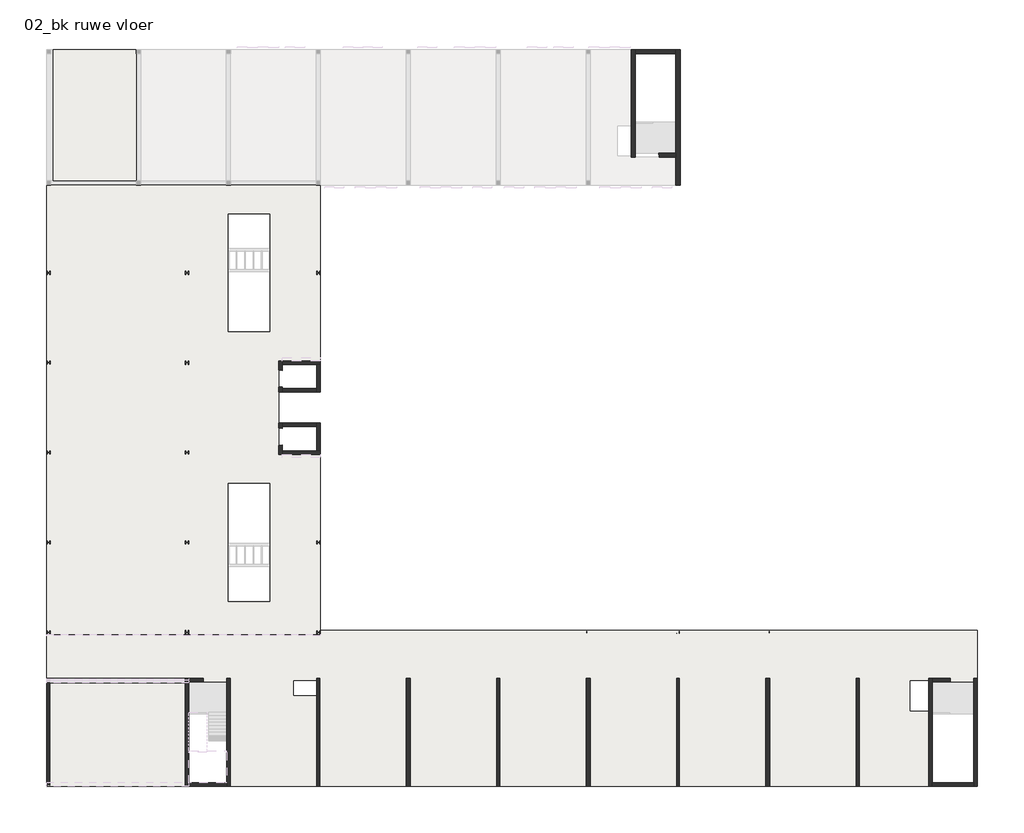
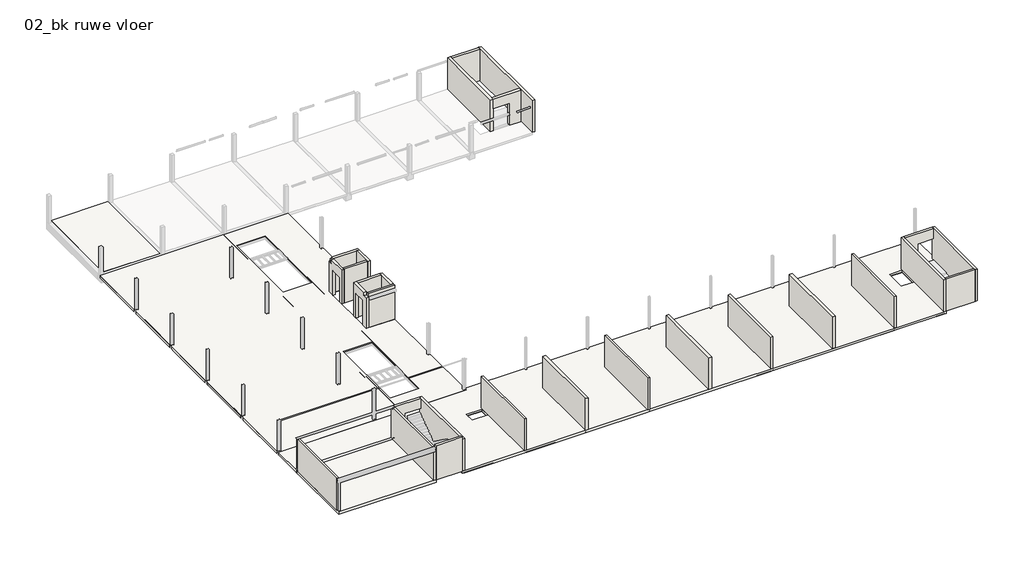
# One storey, part 1 of 3: 28 walls, 20 slabs.
"""IFC4 building model written with IfcOpenShell, lengths in millimetres."""

from ifc_helpers import new_model, si_unit, frame, origin, place, context, project, spatial, polyline, outline, extrude, faceted_brep, element, save

model = new_model("IFC4")

# Units and contexts
model_context = context("Model", 3, world=origin())
ifc_project = project(units=[si_unit("LENGTHUNIT", "METRE", prefix="MILLI")], contexts=[model_context])

# Site, building, storey
site = spatial("IfcSite", under=ifc_project)
building = spatial("IfcBuilding", under=site)
storey = spatial("IfcBuildingStorey", under=building, Name="02_bk ruwe vloer", Elevation=7530.0)

# Slabs
placement = place(None, origin())
element("IfcSlab", 1, ObjectType="NLRS_23_FL_breedplaat 260_gen_rsf", at=placement, inside=storey, context=model_context, shape_type="Brep", body=[
    faceted_brep([(70375.0, -150.0, 7270.0), (70125.0, -150.0, 7270.0), (65150.0, -150.0, 7270.0), (64850.0, -150.0, 7270.0), (58650.0, -150.0, 7270.0), (58350.0, -150.0, 7270.0), (52150.0, -150.0, 7270.0), (51850.0, -150.0, 7270.0), (45650.0, -150.0, 7270.0), (45350.0, -150.0, 7270.0), (39150.0, -150.0, 7270.0), (38850.0, -150.0, 7270.0), (32650.0, -150.0, 7270.0), (32350.0, -150.0, 7270.0), (19625.0, -150.0, 7270.0), (19375.0, -150.0, 7270.0), (19375.0, 7400.0, 7270.0), (16625.0, 7400.0, 7270.0), (16625.0, 7493.0, 7270.0), (16625.0, 7507.0, 7270.0), (6350.0, 7507.0, 7270.0), (6350.0, 10845.0, 7270.0), (26125.0, 10845.0, 7270.0), (26125.0, 11125.0, 7270.0), (73650.0, 11125.0, 7270.0), (73650.0, 7400.0, 7270.0), (73400.0, 7400.0, 7270.0), (70375.0, 7400.0, 7270.0), (6370.0, 7622.0, 7270.0), (19600.0, 7622.0, 7270.0), (19600.0, -130.0, 7270.0), (25875.0, -130.0, 7270.0), (25875.0, 7625.0, 7270.0), (26125.0, 7625.0, 7270.0), (26125.0, -130.0, 7270.0), (32375.0, -130.0, 7270.0), (32375.0, 125.0, 7270.0), (32625.0, 125.0, 7270.0), (32625.0, -130.0, 7270.0), (38875.0, -130.0, 7270.0), (38875.0, 7625.0, 7270.0), (39125.0, 7625.0, 7270.0), (39125.0, -130.0, 7270.0), (45375.0, -130.0, 7270.0), (45375.0, 125.0, 7270.0), (45625.0, 125.0, 7270.0), (45625.0, -130.0, 7270.0), (51875.0, -130.0, 7270.0), (51875.0, 7625.0, 7270.0), (52125.0, 7625.0, 7270.0), (52125.0, -130.0, 7270.0), (58375.0, -130.0, 7270.0), (58375.0, 125.0, 7270.0), (58625.0, 125.0, 7270.0), (58625.0, -130.0, 7270.0), (64875.0, -130.0, 7270.0), (64875.0, 7625.0, 7270.0), (65125.0, 7625.0, 7270.0), (65125.0, -130.0, 7270.0), (70150.0, -130.0, 7270.0), (70150.0, 7625.0, 7270.0), (73630.0, 7625.0, 7270.0), (73630.0, 11105.0, 7270.0), (26145.0, 11105.0, 7270.0), (26145.0, 10761.5, 7270.0), (6370.0, 10761.5, 7270.0), (32375.0, 7625.0, 7270.0), (32625.0, 7625.0, 7270.0), (32625.0, 7375.0, 7270.0), (32375.0, 7375.0, 7270.0), (45375.0, 7625.0, 7270.0), (45625.0, 7625.0, 7270.0), (45625.0, 7375.0, 7270.0), (45375.0, 7375.0, 7270.0), (58375.0, 7625.0, 7270.0), (58625.0, 7625.0, 7270.0), (58625.0, 7375.0, 7270.0), (58375.0, 7375.0, 7270.0), (19375.0, -150.0, 7530.0), (19625.0, -150.0, 7530.0), (32350.0, -150.0, 7530.0), (32650.0, -150.0, 7530.0), (45350.0, -150.0, 7530.0), (45650.0, -150.0, 7530.0), (58350.0, -150.0, 7530.0), (58650.0, -150.0, 7530.0), (70125.0, -150.0, 7530.0), (70375.0, -150.0, 7530.0), (70375.0, 7400.0, 7530.0), (71700.0, 7400.0, 7530.0), (73650.0, 7400.0, 7530.0), (73650.0, 11125.0, 7530.0), (26125.0, 11125.0, 7530.0), (26125.0, 10845.0, 7530.0), (6350.0, 10845.0, 7530.0), (6350.0, 7507.0, 7530.0), (16625.0, 7507.0, 7530.0), (16625.0, 7493.0, 7530.0), (16625.0, 7400.0, 7530.0), (19375.0, 7400.0, 7530.0), (19375.0, 100.0, 7530.0), (24227.5, 6452.0, 7530.0), (24227.5, 7500.0, 7530.0), (25850.0, 7500.0, 7530.0), (25850.0, 6452.0, 7530.0), (68805.0, 5320.0, 7530.0), (68805.0, 7500.0, 7530.0), (70125.0, 7500.0, 7530.0), (70125.0, 5320.0, 7530.0), (6350.0, 10845.0, 7480.0), (26125.0, 10845.0, 7480.0), (19600.0, 7622.0, 7330.0), (6370.0, 7622.0, 7330.0), (6370.0, 10761.5, 7330.0), (26145.0, 10761.5, 7330.0), (26145.0, 11105.0, 7330.0), (73630.0, 11105.0, 7330.0), (73630.0, 7625.0, 7330.0), (70150.0, 7625.0, 7330.0), (70150.0, -130.0, 7330.0), (65125.0, -130.0, 7330.0), (65125.0, 7625.0, 7330.0), (64875.0, 7625.0, 7330.0), (64875.0, -130.0, 7330.0), (58625.0, -130.0, 7330.0), (58625.0, 125.0, 7330.0), (58375.0, 125.0, 7330.0), (58375.0, -130.0, 7330.0), (52125.0, -130.0, 7330.0), (52125.0, 7625.0, 7330.0), (51875.0, 7625.0, 7330.0), (51875.0, -130.0, 7330.0), (45625.0, -130.0, 7330.0), (45625.0, 125.0, 7330.0), (45375.0, 125.0, 7330.0), (45375.0, -130.0, 7330.0), (39125.0, -130.0, 7330.0), (39125.0, 7625.0, 7330.0), (38875.0, 7625.0, 7330.0), (38875.0, -130.0, 7330.0), (32625.0, -130.0, 7330.0), (32625.0, 125.0, 7330.0), (32375.0, 125.0, 7330.0), (32375.0, -130.0, 7330.0), (26125.0, -130.0, 7330.0), (26125.0, 7625.0, 7330.0), (25875.0, 7625.0, 7330.0), (25875.0, -130.0, 7330.0), (19600.0, -130.0, 7330.0), (32625.0, 7625.0, 7330.0), (32375.0, 7625.0, 7330.0), (32375.0, 7375.0, 7330.0), (32625.0, 7375.0, 7330.0), (45625.0, 7625.0, 7330.0), (45375.0, 7625.0, 7330.0), (45375.0, 7375.0, 7330.0), (45625.0, 7375.0, 7330.0), (58625.0, 7625.0, 7330.0), (58375.0, 7625.0, 7330.0), (58375.0, 7375.0, 7330.0), (58625.0, 7375.0, 7330.0), (24227.5, 7500.0, 7330.0), (24227.5, 6452.0, 7330.0), (25850.0, 6452.0, 7330.0), (25850.0, 7500.0, 7330.0), (68805.0, 7500.0, 7330.0), (68805.0, 5320.0, 7330.0), (70125.0, 5320.0, 7330.0), (70125.0, 7500.0, 7330.0)], [[[0, 1, 2, 3, 4, 5, 6, 7, 8, 9, 10, 11, 12, 13, 14, 15, 16, 17, 18, 19, 20, 21, 22, 23, 24, 25, 26, 27], [28, 29, 30, 31, 32, 33, 34, 35, 36, 37, 38, 39, 40, 41, 42, 43, 44, 45, 46, 47, 48, 49, 50, 51, 52, 53, 54, 55, 56, 57, 58, 59, 60, 61, 62, 63, 64, 65]], [[66, 67, 68, 69]], [[70, 71, 72, 73]], [[74, 75, 76, 77]], [[78, 79, 80, 81, 82, 83, 84, 85, 86, 87, 88, 89, 90, 91, 92, 93, 94, 95, 96, 97, 98, 99, 100], [101, 102, 103, 104], [105, 106, 107, 108]], [[15, 14, 13, 12, 11, 10, 9, 8, 7, 6, 5, 4, 3, 2, 1, 0, 87, 86, 85, 84, 83, 82, 81, 80, 79, 78]], [[16, 15, 78, 100, 99]], [[17, 16, 99, 98]], [[17, 98, 97, 96, 19, 18]], [[21, 20, 95, 94, 109]], [[22, 21, 109, 94, 93, 110]], [[23, 22, 110, 93, 92]], [[24, 23, 92, 91]], [[25, 24, 91, 90]], [[27, 26, 25, 90, 89, 88]], [[0, 27, 88, 87]], [[20, 19, 96, 95]], [[111, 112, 113, 114, 115, 116, 117, 118, 119, 120, 121, 122, 123, 124, 125, 126, 127, 128, 129, 130, 131, 132, 133, 134, 135, 136, 137, 138, 139, 140, 141, 142, 143, 144, 145, 146, 147, 148], [149, 150, 151, 152], [153, 154, 155, 156], [157, 158, 159, 160], [161, 162, 163, 164], [165, 166, 167, 168]], [[112, 111, 29, 28]], [[113, 112, 28, 65]], [[114, 113, 65, 64]], [[115, 114, 64, 63]], [[116, 115, 63, 62]], [[117, 116, 62, 61]], [[118, 117, 61, 60]], [[119, 118, 60, 59]], [[120, 119, 59, 58]], [[121, 120, 58, 57]], [[122, 121, 57, 56]], [[123, 122, 56, 55]], [[124, 123, 55, 54]], [[125, 124, 54, 53]], [[126, 125, 53, 52]], [[127, 126, 52, 51]], [[128, 127, 51, 50]], [[129, 128, 50, 49]], [[130, 129, 49, 48]], [[131, 130, 48, 47]], [[132, 131, 47, 46]], [[133, 132, 46, 45]], [[134, 133, 45, 44]], [[135, 134, 44, 43]], [[136, 135, 43, 42]], [[137, 136, 42, 41]], [[138, 137, 41, 40]], [[139, 138, 40, 39]], [[140, 139, 39, 38]], [[141, 140, 38, 37]], [[142, 141, 37, 36]], [[143, 142, 36, 35]], [[144, 143, 35, 34]], [[145, 144, 34, 33]], [[146, 145, 33, 32]], [[147, 146, 32, 31]], [[148, 147, 31, 30]], [[111, 148, 30, 29]], [[150, 149, 67, 66]], [[151, 150, 66, 69]], [[152, 151, 69, 68]], [[149, 152, 68, 67]], [[154, 153, 71, 70]], [[155, 154, 70, 73]], [[156, 155, 73, 72]], [[153, 156, 72, 71]], [[158, 157, 75, 74]], [[159, 158, 74, 77]], [[160, 159, 77, 76]], [[157, 160, 76, 75]], [[102, 101, 162, 161]], [[101, 104, 163, 162]], [[104, 103, 164, 163]], [[103, 102, 161, 164]], [[106, 105, 166, 165]], [[105, 108, 167, 166]], [[108, 107, 168, 167]], [[107, 106, 165, 168]]]),
])
element("IfcSlab", 2, ObjectType="NLRS_23_FL_breedplaat 260_gen_rsf", at=placement, inside=storey, context=model_context, shape_type="Brep", body=[
    faceted_brep([(6830.0, 43680.0, 7270.0), (6830.0, 43800.0, 7270.0), (6830.0, 53150.0, 7270.0), (6950.0, 53150.0, 7270.0), (12700.0, 53150.0, 7270.0), (12820.0, 53150.0, 7270.0), (12820.0, 43800.0, 7270.0), (12820.0, 43680.0, 7270.0), (12725.0, 43775.0, 7270.0), (12725.0, 53140.0, 7270.0), (6925.0, 53140.0, 7270.0), (6925.0, 43775.0, 7270.0), (6830.0, 53150.0, 7530.0), (6830.0, 43680.0, 7530.0), (12820.0, 43680.0, 7530.0), (12820.0, 53150.0, 7530.0), (6925.0, 53140.0, 7330.0), (12725.0, 53140.0, 7330.0), (12725.0, 43775.0, 7330.0), (6925.0, 43775.0, 7330.0)], [[[0, 1, 2, 3, 4, 5, 6, 7], [8, 9, 10, 11]], [[12, 13, 14, 15]], [[2, 1, 0, 13, 12]], [[5, 4, 3, 2, 12, 15]], [[7, 6, 5, 15, 14]], [[0, 7, 14, 13]], [[16, 17, 18, 19]], [[18, 17, 9, 8]], [[19, 18, 8, 11]], [[16, 19, 11, 10]], [[17, 16, 10, 9]]]),
])
element("IfcSlab", 3, ObjectType="NLRS_23_FL_druklaag 70_gen_rsf", at=placement, inside=storey, context=model_context, shape_type="Brep", body=[
    faceted_brep([(6350.0, 43350.0, 7460.0), (26125.0, 43350.0, 7460.0), (26125.0, 43330.0, 7460.0), (26125.0, 37175.0, 7460.0), (26125.0, 37155.0, 7460.0), (22760.0, 37155.0, 7460.0), (22760.0, 36845.0, 7460.0), (26125.0, 36845.0, 7460.0), (26125.0, 36825.0, 7460.0), (26125.0, 30705.0, 7460.0), (26125.0, 30625.0, 7460.0), (23362.3, 30625.0, 7460.0), (23362.3, 30632.0, 7460.0), (6350.0, 30632.0, 7460.0), (6350.0, 30652.0, 7460.0), (6350.0, 36825.0, 7460.0), (6350.0, 36845.0, 7460.0), (19240.0, 36845.0, 7460.0), (19240.0, 37155.0, 7460.0), (6350.0, 37155.0, 7460.0), (6350.0, 37175.0, 7460.0), (6350.0, 43330.0, 7460.0), (22500.0, 32750.0, 7460.0), (22500.0, 41250.0, 7460.0), (19500.0, 41250.0, 7460.0), (19500.0, 32750.0, 7460.0), (23362.3, 23875.0, 7460.0), (26125.0, 23875.0, 7460.0), (26125.0, 23795.0, 7460.0), (26125.0, 17675.0, 7460.0), (26125.0, 17655.0, 7460.0), (26125.0, 17345.0, 7460.0), (26125.0, 17325.0, 7460.0), (26125.0, 11175.0, 7460.0), (26125.0, 11155.0, 7460.0), (6350.0, 11155.0, 7460.0), (6350.0, 11175.0, 7460.0), (6350.0, 17325.0, 7460.0), (6350.0, 17345.0, 7460.0), (19240.0, 17345.0, 7460.0), (19240.0, 17655.0, 7460.0), (6350.0, 17655.0, 7460.0), (6350.0, 17675.0, 7460.0), (6350.0, 23825.0, 7460.0), (6350.0, 23845.0, 7460.0), (19240.0, 23845.0, 7460.0), (19500.0, 23845.0, 7460.0), (22500.0, 23845.0, 7460.0), (22760.0, 23845.0, 7460.0), (23362.3, 23845.0, 7460.0), (22500.0, 21750.0, 7460.0), (19500.0, 21750.0, 7460.0), (19500.0, 13250.0, 7460.0), (22500.0, 13250.0, 7460.0), (19500.0000006, 13240.0, 7460.0), (19500.0000006, 12938.0, 7460.0), (22499.9999994, 12938.0, 7460.0), (22499.9999994, 13240.0, 7460.0), (19500.0000006, 22062.0, 7460.0), (19500.0000006, 21760.0, 7460.0), (22499.9999994, 21760.0, 7460.0), (22499.9999994, 22062.0, 7460.0), (6350.0, 30322.0, 7460.0), (23125.0, 30322.0, 7460.0), (23125.0, 30302.0, 7460.0), (23125.0, 24175.0, 7460.0), (23125.0, 24155.0, 7460.0), (6350.0, 24155.0, 7460.0), (6350.0, 24175.0, 7460.0), (6350.0, 30302.0, 7460.0), (26125.0, 30625.0, 7530.0), (26125.0, 43350.0, 7530.0), (6350.0, 43350.0, 7530.0), (6350.0, 10845.0, 7530.0), (26125.0, 10845.0, 7530.0), (26125.0, 11125.0, 7530.0), (26125.0, 23875.0, 7530.0), (23125.0, 23875.0, 7530.0), (23125.0, 30625.0, 7530.0), (22500.0, 41250.0, 7530.0), (22500.0, 32750.0, 7530.0), (19500.0, 32750.0, 7530.0), (19500.0, 41250.0, 7530.0), (19500.0, 21750.0, 7530.0), (22500.0, 21750.0, 7530.0), (22500.0, 13250.0, 7530.0), (19500.0, 13250.0, 7530.0), (26125.0, 36845.0, 7480.0), (26125.0, 37155.0, 7480.0), (6350.0, 10845.0, 7480.0), (26125.0, 10845.0, 7480.0), (6350.0, 37155.0, 7480.0), (6350.0, 36845.0, 7480.0), (6350.0, 30632.0, 7480.0), (6350.0, 30322.0, 7480.0), (6350.0, 24155.0, 7480.0), (6350.0, 23845.0, 7480.0), (6350.0, 17655.0, 7480.0), (6350.0, 17345.0, 7480.0), (6350.0, 11155.0, 7480.0), (23125.0, 30625.0, 7480.0), (23362.3, 30625.0, 7480.0), (23125.0, 23875.0, 7480.0), (23125.0, 24155.0, 7480.0), (23125.0, 30322.0, 7480.0), (23362.3, 23875.0, 7480.0), (26125.0, 11125.0, 7480.0), (26125.0, 11155.0, 7480.0), (19240.0, 36845.0, 7480.0), (19240.0, 37155.0, 7480.0), (23362.3, 30632.0, 7480.0), (23362.3, 23845.0, 7480.0), (19240.0, 17345.0, 7480.0), (19240.0, 17655.0, 7480.0), (22760.0, 37155.0, 7480.0), (22760.0, 36845.0, 7480.0), (19500.0000006, 13240.0, 7480.0), (19500.0000006, 12938.0, 7480.0), (22499.9999994, 12938.0, 7480.0), (22499.9999994, 13240.0, 7480.0), (19500.0000006, 22062.0, 7480.0), (19500.0000006, 21760.0, 7480.0), (22499.9999994, 21760.0, 7480.0), (22499.9999994, 22062.0, 7480.0)], [[[0, 1, 2, 3, 4, 5, 6, 7, 8, 9, 10, 11, 12, 13, 14, 15, 16, 17, 18, 19, 20, 21], [22, 23, 24, 25]], [[26, 27, 28, 29, 30, 31, 32, 33, 34, 35, 36, 37, 38, 39, 40, 41, 42, 43, 44, 45, 46, 47, 48, 49], [50, 51, 52, 53], [54, 55, 56, 57], [58, 59, 60, 61]], [[62, 63, 64, 65, 66, 67, 68, 69]], [[70, 71, 72, 73, 74, 75, 76, 77, 78], [79, 80, 81, 82], [83, 84, 85, 86]], [[71, 70, 10, 9, 8, 7, 87, 88, 4, 3, 2, 1]], [[74, 73, 89, 90]], [[73, 72, 0, 21, 20, 19, 91, 92, 16, 15, 14, 13, 93, 94, 62, 69, 68, 67, 95, 96, 44, 43, 42, 41, 97, 98, 38, 37, 36, 35, 99, 89]], [[1, 0, 72, 71]], [[70, 78, 100, 101, 11, 10]], [[78, 77, 102, 103, 66, 65, 64, 63, 104, 100]], [[77, 76, 27, 26, 105, 102]], [[27, 76, 75, 74, 90, 106, 107, 34, 33, 32, 31, 30, 29, 28]], [[23, 22, 80, 79]], [[24, 23, 79, 82]], [[25, 24, 82, 81]], [[22, 25, 81, 80]], [[51, 50, 84, 83]], [[52, 51, 83, 86]], [[53, 52, 86, 85]], [[50, 53, 85, 84]], [[108, 109, 18, 17]], [[109, 108, 92, 91]], [[109, 91, 19, 18]], [[92, 108, 17, 16]], [[101, 110, 12, 11]], [[93, 110, 101, 100, 104, 94]], [[110, 93, 13, 12]], [[94, 104, 63, 62]], [[111, 105, 26, 49]], [[111, 96, 95, 103, 102, 105]], [[103, 95, 67, 66]], [[96, 111, 49, 48, 47, 46, 45, 44]], [[112, 113, 40, 39]], [[113, 112, 98, 97]], [[113, 97, 41, 40]], [[98, 112, 39, 38]], [[99, 107, 106, 90, 89]], [[107, 99, 35, 34]], [[114, 115, 6, 5]], [[115, 114, 88, 87]], [[88, 114, 5, 4]], [[115, 87, 7, 6]], [[116, 117, 55, 54]], [[118, 119, 57, 56]], [[117, 116, 119, 118]], [[119, 116, 54, 57]], [[117, 118, 56, 55]], [[120, 121, 59, 58]], [[122, 123, 61, 60]], [[121, 120, 123, 122]], [[121, 122, 60, 59]], [[123, 120, 58, 61]]]),
])
element("IfcSlab", 4, ObjectType="NLRS_23_FL_kanaalplaat 260_gen_rsf", at=placement, inside=storey, context=model_context, shape_type="SweptSolid", body=[
    extrude(outline(polyline([(19240.0, 11175.0), (6350.0, 11175.0), (6350.0, 17325.0), (19240.0, 17325.0), (19240.0, 11175.0)])), frame((0.0, 0.0, 7200.0), z_axis=(0.0, 0.0, 1.0), x_axis=(1.0, 0.0, 0.0)), (0.0, 0.0, 1.0), 260.0),
])
element("IfcSlab", 5, ObjectType="NLRS_23_FL_kanaalplaat 260_gen_rsf", at=placement, inside=storey, context=model_context, shape_type="SweptSolid", body=[
    extrude(outline(polyline([(6350.0, 17675.0), (6350.0, 23825.0), (19240.0, 23825.0), (19240.0, 17675.0), (6350.0, 17675.0)])), frame((0.0, 0.0, 7200.0), z_axis=(0.0, 0.0, 1.0), x_axis=(1.0, 0.0, 0.0)), (0.0, 0.0, 1.0), 260.0),
])
element("IfcSlab", 6, ObjectType="NLRS_23_FL_kanaalplaat 260_gen_rsf", at=placement, inside=storey, context=model_context, shape_type="SweptSolid", body=[
    extrude(outline(polyline([(23125.0, 30302.0), (23125.0, 24175.0), (6350.0, 24175.0), (6350.0, 30302.0), (23125.0, 30302.0)])), frame((0.0, 0.0, 7200.0), z_axis=(0.0, 0.0, 1.0), x_axis=(1.0, 0.0, 0.0)), (0.0, 0.0, 1.0), 260.0),
])
element("IfcSlab", 7, ObjectType="NLRS_23_FL_kanaalplaat 260_gen_rsf", at=placement, inside=storey, context=model_context, shape_type="SweptSolid", body=[
    extrude(outline(polyline([(22500.0, 23825.0), (22500.0, 22082.0), (19500.0, 22082.0), (19500.0, 23825.0), (22500.0, 23825.0)])), frame((0.0, 0.0, 7200.0), z_axis=(0.0, 0.0, 1.0), x_axis=(1.0, 0.0, 0.0)), (0.0, 0.0, 1.0), 260.0),
])
element("IfcSlab", 8, ObjectType="NLRS_23_FL_kanaalplaat 260_gen_rsf", at=placement, inside=storey, context=model_context, shape_type="SweptSolid", body=[
    extrude(outline(polyline([(22500.0, 11182.5), (19500.0, 11182.5), (19500.0, 12918.0), (22500.0, 12918.0), (22500.0, 11182.5)])), frame((0.0, 0.0, 7200.0), z_axis=(0.0, 0.0, 1.0), x_axis=(1.0, 0.0, 0.0)), (0.0, 0.0, 1.0), 260.0),
])
element("IfcSlab", 9, ObjectType="NLRS_23_FL_kanaalplaat 260_gen_rsf", at=placement, inside=storey, context=model_context, shape_type="Brep", body=[
    faceted_brep([(26125.0, 23795.0, 7200.0), (26125.0, 23625.0, 7200.0), (26125.0, 17675.0, 7200.0), (22760.0, 17675.0, 7200.0), (22760.0, 23825.0, 7200.0), (23395.0, 23825.0, 7200.0), (23395.0, 23795.0, 7200.0), (26125.0, 23795.0, 7460.0), (23395.0, 23795.0, 7460.0), (23395.0, 23825.0, 7460.0), (22760.0, 23825.0, 7460.0), (22760.0, 17675.0, 7460.0), (26125.0, 17675.0, 7460.0)], [[[0, 1, 2, 3, 4, 5, 6]], [[7, 8, 9, 10, 11, 12]], [[2, 1, 0, 7, 12]], [[3, 2, 12, 11]], [[4, 3, 11, 10]], [[5, 4, 10, 9]], [[6, 5, 9, 8]], [[0, 6, 8, 7]]]),
])
element("IfcSlab", 10, ObjectType="NLRS_23_FL_kanaalplaat 260_gen_rsf", at=placement, inside=storey, context=model_context, shape_type="SweptSolid", body=[
    extrude(outline(polyline([(22760.0, 11175.0), (22760.0, 17325.0), (26125.0, 17325.0), (26125.0, 11175.0), (22760.0, 11175.0)])), frame((0.0, 0.0, 7200.0), z_axis=(0.0, 0.0, 1.0), x_axis=(1.0, 0.0, 0.0)), (0.0, 0.0, 1.0), 260.0),
])
element("IfcSlab", 11, ObjectType="NLRS_23_FL_kanaalplaat 260_gen_rsf", at=placement, inside=storey, context=model_context, shape_type="Brep", body=[
    faceted_brep([(19240.0, 43330.0, 7200.0), (19240.0, 37175.0, 7200.0), (6350.0, 37175.0, 7200.0), (6350.0, 43200.0, 7200.0), (6350.0, 43330.0, 7200.0), (19240.0, 43330.0, 7460.0), (6350.0, 43330.0, 7460.0), (6350.0, 37175.0, 7460.0), (19240.0, 37175.0, 7460.0)], [[[0, 1, 2, 3, 4]], [[5, 6, 7, 8]], [[0, 4, 6, 5]], [[4, 3, 2, 7, 6]], [[2, 1, 8, 7]], [[1, 0, 5, 8]]]),
])
element("IfcSlab", 12, ObjectType="NLRS_23_FL_kanaalplaat 260_gen_rsf", at=placement, inside=storey, context=model_context, shape_type="SweptSolid", body=[
    extrude(outline(polyline([(6350.0, 36825.0), (19240.0, 36825.0), (19240.0, 30652.0), (6350.0, 30652.0), (6350.0, 36825.0)])), frame((0.0, 0.0, 7200.0), z_axis=(0.0, 0.0, 1.0), x_axis=(1.0, 0.0, 0.0)), (0.0, 0.0, 1.0), 260.0),
])
element("IfcSlab", 13, ObjectType="NLRS_23_FL_kanaalplaat 260_gen_rsf", at=placement, inside=storey, context=model_context, shape_type="SweptSolid", body=[
    extrude(outline(polyline([(22500.0, 30652.0), (19500.0, 30652.0), (19500.0, 32418.0), (22500.0, 32418.0), (22500.0, 30652.0)])), frame((0.0, 0.0, 7200.0), z_axis=(0.0, 0.0, 1.0), x_axis=(1.0, 0.0, 0.0)), (0.0, 0.0, 1.0), 260.0),
])
element("IfcSlab", 14, ObjectType="NLRS_23_FL_kanaalplaat 260_gen_rsf", at=placement, inside=storey, context=model_context, shape_type="SweptSolid", body=[
    extrude(outline(polyline([(22500.0, 43330.0), (22500.0, 41605.0), (19500.0, 41605.0), (19500.0, 43330.0), (22500.0, 43330.0)])), frame((0.0, 0.0, 7200.0), z_axis=(0.0, 0.0, 1.0), x_axis=(1.0, 0.0, 0.0)), (0.0, 0.0, 1.0), 260.0),
])
element("IfcSlab", 15, ObjectType="NLRS_23_FL_kanaalplaat 260_gen_rsf", at=placement, inside=storey, context=model_context, shape_type="Brep", body=[
    faceted_brep([(26125.0, 30705.0, 7200.0), (23395.0, 30705.0, 7200.0), (23395.0, 30652.0, 7200.0), (22760.0, 30652.0, 7200.0), (22760.0, 36825.0, 7200.0), (26125.0, 36825.0, 7200.0), (26125.0, 30875.0, 7200.0), (26125.0, 30705.0, 7460.0), (26125.0, 36825.0, 7460.0), (22760.0, 36825.0, 7460.0), (22760.0, 30652.0, 7460.0), (23395.0, 30652.0, 7460.0), (23395.0, 30705.0, 7460.0)], [[[0, 1, 2, 3, 4, 5, 6]], [[7, 8, 9, 10, 11, 12]], [[0, 6, 5, 8, 7]], [[5, 4, 9, 8]], [[4, 3, 10, 9]], [[3, 2, 11, 10]], [[2, 1, 12, 11]], [[1, 0, 7, 12]]]),
])
element("IfcSlab", 16, ObjectType="NLRS_23_FL_kanaalplaat 260_gen_rsf", at=placement, inside=storey, context=model_context, shape_type="Brep", body=[
    faceted_brep([(22760.0, 43330.0, 7200.0), (26125.0, 43330.0, 7200.0), (26125.0, 43200.0, 7200.0), (26125.0, 37175.0, 7200.0), (22760.0, 37175.0, 7200.0), (22760.0, 43330.0, 7460.0), (22760.0, 37175.0, 7460.0), (26125.0, 37175.0, 7460.0), (26125.0, 43330.0, 7460.0)], [[[0, 1, 2, 3, 4]], [[5, 6, 7, 8]], [[0, 4, 6, 5]], [[4, 3, 7, 6]], [[3, 2, 1, 8, 7]], [[1, 0, 5, 8]]]),
])
element("IfcSlab", 17, ObjectType="NLRS_23_FL_breedplaat 260_gen_rsf", at=placement, inside=storey, context=model_context, shape_type="Brep", body=[
    faceted_brep([(6350.0, -150.0, 7270.0), (6350.0, 7493.0, 7270.0), (16625.0, 7493.0, 7270.0), (16625.0, 7330.0, 7270.0), (16625.0, 170.0, 7270.0), (16625.0, -150.0, 7270.0), (16400.0, 125.0, 7270.0), (16400.0, 7378.0, 7270.0), (6539.0, 7378.0, 7270.0), (6539.0, 125.0, 7270.0), (6350.0, 7493.0, 7530.0), (6350.0, -150.0, 7530.0), (16375.0, -150.0, 7530.0), (16625.0, -150.0, 7530.0), (16625.0, 100.0, 7530.0), (16625.0, 7493.0, 7530.0), (6539.0, 7378.0, 7330.0), (16400.0, 7378.0, 7330.0), (16400.0, 125.0, 7330.0), (6539.0, 125.0, 7330.0)], [[[0, 1, 2, 3, 4, 5], [6, 7, 8, 9]], [[10, 11, 12, 13, 14, 15]], [[1, 0, 11, 10]], [[2, 1, 10, 15]], [[5, 4, 3, 2, 15, 14, 13]], [[0, 5, 13, 12, 11]], [[16, 17, 18, 19]], [[18, 17, 7, 6]], [[19, 18, 6, 9]], [[16, 19, 9, 8]], [[17, 16, 8, 7]]]),
])
element("IfcSlab", 18, ObjectType="NLRS_23_FL_breedplaat schil 60_gen_rsf", at=placement, inside=storey, context=model_context, shape_type="SweptSolid", body=[
    extrude(outline(polyline([(19600.0, 7622.0), (6370.0, 7622.0), (6370.0, 10761.5), (26145.0, 10761.5), (26145.0, 11105.0), (73630.0, 11105.0), (73630.0, 7625.0), (70150.0, 7625.0), (70150.0, -130.0), (65125.0, -130.0), (65125.0, 7625.0), (64875.0, 7625.0), (64875.0, -130.0), (58625.0, -130.0), (58625.0, 125.0), (58375.0, 125.0), (58375.0, -130.0), (52125.0, -130.0), (52125.0, 7625.0), (51875.0, 7625.0), (51875.0, -130.0), (45625.0, -130.0), (45625.0, 125.0), (45375.0, 125.0), (45375.0, -130.0), (39125.0, -130.0), (39125.0, 7625.0), (38875.0, 7625.0), (38875.0, -130.0), (32625.0, -130.0), (32625.0, 125.0), (32375.0, 125.0), (32375.0, -130.0), (26125.0, -130.0), (26125.0, 7625.0), (25875.0, 7625.0), (25875.0, -130.0), (19600.0, -130.0), (19600.0, 7622.0)]), holes=[polyline([(32625.0, 7625.0), (32375.0, 7625.0), (32375.0, 7375.0), (32625.0, 7375.0), (32625.0, 7625.0)]), polyline([(45625.0, 7625.0), (45375.0, 7625.0), (45375.0, 7375.0), (45625.0, 7375.0), (45625.0, 7625.0)]), polyline([(58625.0, 7625.0), (58375.0, 7625.0), (58375.0, 7375.0), (58625.0, 7375.0), (58625.0, 7625.0)]), polyline([(24227.5, 7500.0), (24227.5, 6452.0), (25850.0, 6452.0), (25850.0, 7500.0), (24227.5, 7500.0)]), polyline([(68805.0, 7500.0), (68805.0, 5320.0), (70125.0, 5320.0), (70125.0, 7500.0), (68805.0, 7500.0)])]), frame((0.0, 0.0, 7270.0), z_axis=(0.0, 0.0, 1.0), x_axis=(1.0, 0.0, 0.0)), (0.0, 0.0, 1.0), 60.0),
])
element("IfcSlab", 19, ObjectType="NLRS_23_FL_breedplaat schil 60_gen_rsf", at=placement, inside=storey, context=model_context, shape_type="SweptSolid", body=[
    extrude(outline(polyline([(16400.0, 7378.0), (16400.0, 125.0), (6539.0, 125.0), (6539.0, 7378.0), (16400.0, 7378.0)])), frame((0.0, 0.0, 7270.0), z_axis=(0.0, 0.0, 1.0), x_axis=(1.0, 0.0, 0.0)), (0.0, 0.0, 1.0), 60.0),
])
element("IfcSlab", 20, ObjectType="NLRS_23_FL_breedplaat schil 60_gen_rsf", at=placement, inside=storey, context=model_context, shape_type="SweptSolid", body=[
    extrude(outline(polyline([(12725.0, 53140.0), (12725.0, 43775.0), (6925.0, 43775.0), (6925.0, 53140.0), (12725.0, 53140.0)])), frame((0.0, 0.0, 7270.0), z_axis=(0.0, 0.0, 1.0), x_axis=(1.0, 0.0, 0.0)), (0.0, 0.0, 1.0), 60.0),
])

# Walls
element("IfcWall", 21, ObjectType="NLRS_22_WA_beton ihw 250_gen_rsf", at=placement, inside=storey, context=model_context, shape_type="Brep", body=[
    faceted_brep([(19625.0, -150.0, 7530.0), (19625.0, 7650.0, 7530.0), (19625.0, 7650.0, 11070.0), (19625.0, -150.0, 11070.0), (19375.0, -150.0, 7530.0), (19375.0, -150.0, 11070.0), (19375.0, 7400.0, 11070.0), (19375.0, 7650.0, 11070.0), (19375.0, 7650.0, 9970.0), (19375.0, 7650.0, 7530.0), (19375.0, 7400.0, 7530.0), (19375.0, 100.0, 7530.0)], [[[0, 1, 2, 3]], [[4, 5, 6, 7, 8, 9, 10, 11]], [[1, 0, 4, 11, 10, 9]], [[2, 1, 9, 8, 7]], [[3, 2, 7, 6, 5]], [[0, 3, 5, 4]]]),
])
element("IfcWall", 22, ObjectType="NLRS_22_WA_beton ihw 250_gen_rsf", at=placement, inside=storey, context=model_context, shape_type="Brep", body=[
    faceted_brep([(16625.0, -150.0, 7530.0), (16625.0, 100.0, 7530.0), (16625.0, 7400.0, 7530.0), (16625.0, 7493.0, 7530.0), (16625.0, 7650.0, 7530.0), (16625.0, 7650.0, 10940.0), (16625.0, 7330.0, 10940.0), (16625.0, 7330.0, 11070.0), (16625.0, 170.0, 11070.0), (16625.0, 170.0, 10680.0), (16625.0, -150.0, 10680.0), (16375.0, -150.0, 7530.0), (16375.0, -150.0, 10680.0), (16375.0, 170.0, 10680.0), (16375.0, 170.0, 11070.0), (16375.0, 7330.0, 11070.0), (16375.0, 7330.0, 10940.0), (16375.0, 7650.0, 10940.0), (16375.0, 7650.0, 7530.0)], [[[0, 1, 2, 3, 4, 5, 6, 7, 8, 9, 10]], [[11, 12, 13, 14, 15, 16, 17, 18]], [[4, 3, 2, 1, 0, 11, 18]], [[5, 4, 18, 17]], [[8, 7, 15, 14]], [[0, 10, 12, 11]], [[9, 8, 14, 13]], [[10, 9, 13, 12]], [[6, 5, 17, 16]], [[7, 6, 16, 15]]]),
])
element("IfcWall", 23, ObjectType="NLRS_22_WA_kalkzandsteen CS12 214_gen_rsf", at=placement, inside=storey, context=model_context, shape_type="SweptSolid", body=[
    extrude(outline(polyline([(26107.0, 7650.0), (26107.0, -150.0), (25893.0, -150.0), (25893.0, 7650.0), (26107.0, 7650.0)])), frame((0.0, 0.0, 7530.0), z_axis=(0.0, 0.0, 1.0), x_axis=(1.0, 0.0, 0.0)), (0.0, 0.0, 1.0), 3540.0),
])
element("IfcWall", 24, ObjectType="NLRS_22_WA_beton ihw 300_gen_rsf", at=placement, inside=storey, context=model_context, shape_type="SweptSolid", body=[
    extrude(outline(polyline([(32650.0, 7650.0), (32650.0, -150.0), (32350.0, -150.0), (32350.0, 7650.0), (32650.0, 7650.0)])), frame((0.0, 0.0, 7530.0), z_axis=(0.0, 0.0, 1.0), x_axis=(1.0, 0.0, 0.0)), (0.0, 0.0, 1.0), 3540.0),
])
element("IfcWall", 25, ObjectType="NLRS_22_WA_kalkzandsteen CS12 214_gen_rsf", at=placement, inside=storey, context=model_context, shape_type="SweptSolid", body=[
    extrude(outline(polyline([(39107.0, 7650.0), (39107.0, -150.0), (38893.0, -150.0), (38893.0, 7650.0), (39107.0, 7650.0)])), frame((0.0, 0.0, 7530.0), z_axis=(0.0, 0.0, 1.0), x_axis=(1.0, 0.0, 0.0)), (0.0, 0.0, 1.0), 3540.0),
])
element("IfcWall", 26, ObjectType="NLRS_22_WA_beton ihw 300_gen_rsf", at=placement, inside=storey, context=model_context, shape_type="SweptSolid", body=[
    extrude(outline(polyline([(45650.0, 7650.0), (45650.0, -150.0), (45350.0, -150.0), (45350.0, 7650.0), (45650.0, 7650.0)])), frame((0.0, 0.0, 7530.0), z_axis=(0.0, 0.0, 1.0), x_axis=(1.0, 0.0, 0.0)), (0.0, 0.0, 1.0), 3540.0),
])
element("IfcWall", 27, ObjectType="NLRS_22_WA_kalkzandsteen CS12 214_gen_rsf", at=placement, inside=storey, context=model_context, shape_type="SweptSolid", body=[
    extrude(outline(polyline([(52107.0, 7650.0), (52107.0, -150.0), (51893.0, -150.0), (51893.0, 7650.0), (52107.0, 7650.0)])), frame((0.0, 0.0, 7530.0), z_axis=(0.0, 0.0, 1.0), x_axis=(1.0, 0.0, 0.0)), (0.0, 0.0, 1.0), 3540.0),
])
element("IfcWall", 28, ObjectType="NLRS_22_WA_beton ihw 300_gen_rsf", at=placement, inside=storey, context=model_context, shape_type="SweptSolid", body=[
    extrude(outline(polyline([(58650.0, 7650.0), (58650.0, -150.0), (58350.0, -150.0), (58350.0, 7650.0), (58650.0, 7650.0)])), frame((0.0, 0.0, 7530.0), z_axis=(0.0, 0.0, 1.0), x_axis=(1.0, 0.0, 0.0)), (0.0, 0.0, 1.0), 3540.0),
])
element("IfcWall", 29, ObjectType="NLRS_22_WA_kalkzandsteen CS12 214_gen_rsf", at=placement, inside=storey, context=model_context, shape_type="SweptSolid", body=[
    extrude(outline(polyline([(65107.0, 7650.0), (65107.0, -150.0), (64893.0, -150.0), (64893.0, 7650.0), (65107.0, 7650.0)])), frame((0.0, 0.0, 7530.0), z_axis=(0.0, 0.0, 1.0), x_axis=(1.0, 0.0, 0.0)), (0.0, 0.0, 1.0), 3540.0),
])
element("IfcWall", 30, ObjectType="NLRS_21_WA_beton ihw 250_gen_rsf", at=placement, inside=storey, context=model_context, shape_type="Brep", body=[
    faceted_brep([(73650.0, -150.0, 7530.0), (73650.0, 7400.0, 7530.0), (73650.0, 7650.0, 7530.0), (73650.0, 7650.0, 11070.0), (73650.0, -150.0, 11070.0), (73400.0, -150.0, 7530.0), (73400.0, -150.0, 11070.0), (73400.0, 100.0, 11070.0), (73400.0, 7400.0, 11070.0), (73400.0, 7650.0, 11070.0), (73400.0, 7650.0, 9970.0), (73400.0, 7650.0, 7530.0), (73400.0, 7400.0, 7530.0), (73400.0, 100.0, 7530.0)], [[[0, 1, 2, 3, 4]], [[5, 6, 7, 8, 9, 10, 11, 12, 13]], [[2, 1, 0, 5, 13, 12, 11]], [[3, 2, 11, 10, 9]], [[4, 3, 9, 8, 7, 6]], [[0, 4, 6, 5]]]),
])
element("IfcWall", 31, ObjectType="NLRS_21_WA_kalkzandsteen CS12 214_gen_rsf", at=placement, inside=storey, context=model_context, shape_type="SweptSolid", body=[
    extrude(outline(polyline([(6564.0, 7330.0), (6564.0, 170.0), (6350.0, 170.0), (6350.0, 7330.0), (6564.0, 7330.0)])), frame((0.0, 0.0, 7530.0), z_axis=(0.0, 0.0, 1.0), x_axis=(1.0, 0.0, 0.0)), (0.0, 0.0, 1.0), 3540.0),
])
element("IfcWall", 32, ObjectType="NLRS_21_WA_beton ihw 250_gen_rsf", at=placement, inside=storey, context=model_context, shape_type="Brep", body=[
    faceted_brep([(16625.0, -150.0, 7530.0), (19375.0, -150.0, 7530.0), (19375.0, -150.0, 11070.0), (19375.0, -150.0, 11330.0), (16625.0, -150.0, 11330.0), (16625.0, -150.0, 11070.0), (16625.0, -150.0, 10680.0), (19375.0, 100.0, 7530.0), (16625.0, 100.0, 7530.0), (16625.0, 100.0, 11330.0), (19375.0, 100.0, 11330.0), (19375.0, 100.0, 11070.0)], [[[0, 1, 2, 3, 4, 5, 6]], [[7, 8, 9, 10, 11]], [[1, 0, 8, 7]], [[1, 7, 11, 10, 3, 2]], [[4, 3, 10, 9]], [[0, 6, 5, 4, 9, 8]]]),
])
element("IfcWall", 33, ObjectType="NLRS_22_WA_beton ihw 250_gen_rsf", at=placement, inside=storey, context=model_context, shape_type="Brep", body=[
    faceted_brep([(19375.0, 7400.0, 11070.0), (16625.0, 7400.0, 11070.0), (16625.0, 7400.0, 7530.0), (17675.0, 7400.0, 7530.0), (17675.0, 7400.0, 9970.0), (19375.0, 7400.0, 9970.0), (16625.0, 7650.0, 11070.0), (19375.0, 7650.0, 11070.0), (19375.0, 7650.0, 9970.0), (17675.0, 7650.0, 9970.0), (17675.0, 7650.0, 7530.0), (16625.0, 7650.0, 7530.0), (16625.0, 7650.0, 10940.0)], [[[0, 1, 2, 3, 4, 5]], [[6, 7, 8, 9, 10, 11, 12]], [[2, 11, 10, 3]], [[7, 0, 5, 8]], [[1, 0, 7, 6]], [[2, 1, 6, 12, 11]], [[9, 4, 3, 10]], [[4, 9, 8, 5]]]),
])
element("IfcWall", 34, ObjectType="NLRS_22_WA_beton ihw 250_gen_rsf", at=placement, inside=storey, context=model_context, shape_type="Brep", body=[
    faceted_brep([(70375.0, -150.0, 7530.0), (70375.0, 100.0, 7530.0), (70375.0, 7400.0, 7530.0), (70375.0, 7650.0, 7530.0), (70375.0, 7650.0, 11070.0), (70375.0, 7400.0, 11070.0), (70375.0, 100.0, 11070.0), (70375.0, -150.0, 11070.0), (70125.0, -150.0, 7530.0), (70125.0, -150.0, 11070.0), (70125.0, 7650.0, 11070.0), (70125.0, 7650.0, 7530.0), (70125.0, 7500.0, 7530.0), (70125.0, 5320.0, 7530.0)], [[[0, 1, 2, 3, 4, 5, 6, 7]], [[8, 9, 10, 11, 12, 13]], [[3, 2, 1, 0, 8, 13, 12, 11]], [[4, 3, 11, 10]], [[7, 6, 5, 4, 10, 9]], [[0, 7, 9, 8]]]),
])
element("IfcWall", 35, ObjectType="NLRS_21_WA_beton ihw 250_gen_rsf", at=placement, inside=storey, context=model_context, shape_type="SweptSolid", body=[
    extrude(outline(polyline([(73400.0, -150.0), (70375.0, -150.0), (70375.0, 100.0), (73400.0, 100.0), (73400.0, -150.0)])), frame((0.0, 0.0, 7530.0), z_axis=(0.0, 0.0, 1.0), x_axis=(1.0, 0.0, 0.0)), (0.0, 0.0, 1.0), 3540.0),
])
element("IfcWall", 36, ObjectType="NLRS_22_WA_beton ihw 250_gen_rsf", at=placement, inside=storey, context=model_context, shape_type="SweptSolid", body=[
    extrude(outline(polyline([(11070.0, 73400.0), (11070.0, 70375.0), (7530.0, 70375.0), (7530.0, 71700.0), (9970.0, 71700.0), (9970.0, 73400.0), (11070.0, 73400.0)])), frame((0.0, 7400.0, 0.0), z_axis=(0.0, 1.0, 0.0), x_axis=(0.0, 0.0, 1.0)), (0.0, 0.0, 1.0), 250.0),
])
element("IfcWall", 37, ObjectType="NLRS_22_WA_beton prefab 300_gen_rsf", at=placement, inside=storey, context=model_context, shape_type="SweptSolid", body=[
    extrude(outline(polyline([(48905.0, 53150.0), (48905.0, 45350.0), (48605.0, 45350.0), (48605.0, 53150.0), (48905.0, 53150.0)])), frame((0.0, 0.0, 7550.0), z_axis=(0.0, 0.0, 1.0), x_axis=(1.0, 0.0, 0.0)), (0.0, 0.0, 1.0), 3520.0),
])
element("IfcWall", 38, ObjectType="NLRS_21_WA_beton prefab 300_gen_rsf", at=placement, inside=storey, context=model_context, shape_type="SweptSolid", body=[
    extrude(outline(polyline([(52150.0, 53150.0), (52150.0, 43350.0), (51850.0, 43350.0), (51850.0, 53150.0), (52150.0, 53150.0)])), frame((0.0, 0.0, 7550.0), z_axis=(0.0, 0.0, 1.0), x_axis=(1.0, 0.0, 0.0)), (0.0, 0.0, 1.0), 3520.0),
])
element("IfcWall", 39, ObjectType="NLRS_21_WA_beton prefab 300_gen_rsf", at=placement, inside=storey, context=model_context, shape_type="SweptSolid", body=[
    extrude(outline(polyline([(48925.0, 53150.0), (51830.0, 53150.0), (51830.0, 52850.0), (48925.0, 52850.0), (48925.0, 53150.0)])), frame((0.0, 0.0, 7550.0), z_axis=(0.0, 0.0, 1.0), x_axis=(1.0, 0.0, 0.0)), (0.0, 0.0, 1.0), 3520.0),
])
element("IfcWall", 40, ObjectType="NLRS_22_WA_beton prefab 300_gen_rsf", at=placement, inside=storey, context=model_context, shape_type="Brep", body=[
    faceted_brep([(48925.0, 45650.0, 11070.0), (51830.0, 45650.0, 11070.0), (51830.0, 45650.0, 7550.0), (50625.0, 45650.0, 7550.0), (50625.0, 45650.0, 9970.0), (48925.0, 45650.0, 9970.0), (51830.0, 45350.0, 11070.0), (48925.0, 45350.0, 11070.0), (48925.0, 45350.0, 10000.0), (50655.0, 45350.0, 10000.0), (50655.0, 45350.0, 7550.0), (51830.0, 45350.0, 7550.0)], [[[0, 1, 2, 3, 4, 5]], [[6, 7, 8, 9, 10, 11]], [[2, 11, 10, 3]], [[7, 0, 5, 8]], [[1, 0, 7, 6]], [[2, 1, 6, 11]], [[9, 4, 3, 10]], [[4, 9, 8, 5]]]),
])
element("IfcWall", 41, ObjectType="NLRS_22_WA_beton prefab 250_gen_rsf", at=placement, inside=storey, context=model_context, shape_type="Brep", body=[
    faceted_brep([(26125.0, 30625.0, 7550.0), (23395.0, 30625.0, 7550.0), (23395.0, 30625.0, 10750.0), (23395.0, 30625.0, 11000.0), (23395.0, 30625.0, 11330.0), (26125.0, 30625.0, 11330.0), (26125.0, 30625.0, 11000.0), (26125.0, 30625.0, 10750.0), (26125.0, 30375.0, 7550.0), (26125.0, 30375.0, 11330.0), (23395.0, 30375.0, 11330.0), (23395.0, 30375.0, 7550.0)], [[[0, 1, 2, 3, 4, 5, 6, 7]], [[8, 9, 10, 11]], [[1, 0, 8, 11]], [[4, 3, 2, 1, 11, 10]], [[5, 4, 10, 9]], [[0, 7, 6, 5, 9, 8]]]),
])
element("IfcWall", 42, ObjectType="NLRS_22_WA_beton prefab 250_gen_rsf", at=placement, inside=storey, context=model_context, shape_type="Brep", body=[
    faceted_brep([(23125.0, 28375.0, 7550.0), (23125.0, 28375.0, 11330.0), (23125.0, 30231.5, 11330.0), (23125.0, 30231.5, 10955.0), (23125.0, 30625.0, 10955.0), (23125.0, 30625.0, 7550.0), (23125.0, 29973.0, 7550.0), (23125.0, 29973.0, 10305.0), (23125.0, 28723.0, 10305.0), (23125.0, 28723.0, 7550.0), (23375.0, 28375.0, 11330.0), (23375.0, 28375.0, 7550.0), (23375.0, 28748.0, 7550.0), (23375.0, 28748.0, 10280.0), (23375.0, 29948.0, 10280.0), (23375.0, 29948.0, 7550.0), (23375.0, 30625.0, 7550.0), (23375.0, 30625.0, 10955.0), (23375.0, 30231.5, 10955.0), (23375.0, 30231.5, 11330.0)], [[[0, 1, 2, 3, 4, 5, 6, 7, 8, 9]], [[10, 11, 12, 13, 14, 15, 16, 17, 18, 19]], [[11, 0, 9, 12]], [[5, 16, 15, 6]], [[1, 0, 11, 10]], [[2, 1, 10, 19]], [[5, 4, 17, 16]], [[3, 2, 19, 18]], [[4, 3, 18, 17]], [[14, 7, 6, 15]], [[8, 13, 12, 9]], [[7, 14, 13, 8]]]),
])
element("IfcWall", 43, ObjectType="NLRS_22_WA_beton prefab 250_gen_rsf", at=placement, inside=storey, context=model_context, shape_type="SweptSolid", body=[
    extrude(outline(polyline([(25855.0, 28375.0), (23395.0, 28375.0), (23395.0, 28625.0), (25855.0, 28625.0), (25855.0, 28375.0)])), frame((0.0, 0.0, 7550.0), z_axis=(0.0, 0.0, 1.0), x_axis=(1.0, 0.0, 0.0)), (0.0, 0.0, 1.0), 3780.0),
])
element("IfcWall", 44, ObjectType="NLRS_21_WA_beton prefab 250_gen_rsf", at=placement, inside=storey, context=model_context, shape_type="SweptSolid", body=[
    extrude(outline(polyline([(26125.0, 30355.0), (26125.0, 28375.0), (25875.0, 28375.0), (25875.0, 30355.0), (26125.0, 30355.0)])), frame((0.0, 0.0, 7550.0), z_axis=(0.0, 0.0, 1.0), x_axis=(1.0, 0.0, 0.0)), (0.0, 0.0, 1.0), 3780.0),
])
element("IfcWall", 45, ObjectType="NLRS_22_WA_beton prefab 250_gen_rsf", at=placement, inside=storey, context=model_context, shape_type="SweptSolid", body=[
    extrude(outline(polyline([(23395.0, 26125.0), (25855.0, 26125.0), (25855.0, 25875.0), (23395.0, 25875.0), (23395.0, 26125.0)])), frame((0.0, 0.0, 7550.0), z_axis=(0.0, 0.0, 1.0), x_axis=(1.0, 0.0, 0.0)), (0.0, 0.0, 1.0), 3780.0),
])
element("IfcWall", 46, ObjectType="NLRS_22_WA_beton prefab 250_gen_rsf", at=placement, inside=storey, context=model_context, shape_type="Brep", body=[
    faceted_brep([(23125.0, 23875.0, 7550.0), (23125.0, 23875.0, 10955.0), (23125.0, 24291.5, 10955.0), (23125.0, 24291.5, 11330.0), (23125.0, 26125.0, 11330.0), (23125.0, 26125.0, 7550.0), (23125.0, 25777.0, 7550.0), (23125.0, 25777.0, 10305.0), (23125.0, 24527.0, 10305.0), (23125.0, 24527.0, 7550.0), (23375.0, 23875.0, 10955.0), (23375.0, 23875.0, 7550.0), (23375.0, 24552.0, 7550.0), (23375.0, 24552.0, 10280.0), (23375.0, 25752.0, 10280.0), (23375.0, 25752.0, 7550.0), (23375.0, 26125.0, 7550.0), (23375.0, 26125.0, 11330.0), (23375.0, 24291.5, 11330.0), (23375.0, 24291.5, 10955.0)], [[[0, 1, 2, 3, 4, 5, 6, 7, 8, 9]], [[10, 11, 12, 13, 14, 15, 16, 17, 18, 19]], [[11, 0, 9, 12]], [[5, 16, 15, 6]], [[1, 0, 11, 10]], [[4, 3, 18, 17]], [[5, 4, 17, 16]], [[2, 1, 10, 19]], [[3, 2, 19, 18]], [[14, 7, 6, 15]], [[8, 13, 12, 9]], [[7, 14, 13, 8]]]),
])
element("IfcWall", 47, ObjectType="NLRS_22_WA_beton prefab 250_gen_rsf", at=placement, inside=storey, context=model_context, shape_type="Brep", body=[
    faceted_brep([(23395.0, 23875.0, 7550.0), (26125.0, 23875.0, 7550.0), (26125.0, 23875.0, 10750.0), (26125.0, 23875.0, 11000.0), (26125.0, 23875.0, 11330.0), (23395.0, 23875.0, 11330.0), (23395.0, 23875.0, 11000.0), (23395.0, 23875.0, 10750.0), (23395.0, 24125.0, 7550.0), (23395.0, 24125.0, 11330.0), (26125.0, 24125.0, 11330.0), (26125.0, 24125.0, 7550.0)], [[[0, 1, 2, 3, 4, 5, 6, 7]], [[8, 9, 10, 11]], [[1, 0, 8, 11]], [[4, 3, 2, 1, 11, 10]], [[5, 4, 10, 9]], [[0, 7, 6, 5, 9, 8]]]),
])
element("IfcWall", 48, ObjectType="NLRS_21_WA_beton prefab 250_gen_rsf", at=placement, inside=storey, context=model_context, shape_type="SweptSolid", body=[
    extrude(outline(polyline([(26125.0, 26125.0), (26125.0, 24145.0), (25875.0, 24145.0), (25875.0, 26125.0), (26125.0, 26125.0)])), frame((0.0, 0.0, 7550.0), z_axis=(0.0, 0.0, 1.0), x_axis=(1.0, 0.0, 0.0)), (0.0, 0.0, 1.0), 3780.0),
])

save(model, "model.ifc")

# Revit data of these elements
# Type "NLRS_23_FL_breedplaat 260_gen_rsf"
#   Keynote = ""
#   Export Type to IFC As = "IfcSlab"
#   Type IfcGUID = "2ajLwCSRTE_9I1Spg4tpL_"
#   Type Comments = "d=260mm"
#   Description = "breedplaatvloer, vrijdragend"
#   Assembly Code = "23.21"
#   Function = 1
#   Layers, outside or top first: 260 mm "NLRS_f2_beton ihwg_gen_rsf" (function 1)
# Type "NLRS_23_FL_druklaag 70_gen_rsf"
#   Keynote = ""
#   Export Type to IFC As = "IfcSlab"
#   Type IfcGUID = "2GRbcre991teoKeCLB8MGP"
#   Type Comments = "d=70mm"
#   Description = "druklaag"
#   Assembly Code = "23.21"
#   Function = 1
#   Layers, outside or top first: 70 mm "NLRS_f2_beton ihwg_gen_rsf" (function 1)
# Type "NLRS_23_FL_kanaalplaat 260_gen_rsf"
#   Keynote = ""
#   Export Type to IFC As = "IfcSlab"
#   Type IfcGUID = "3PAoVTCyX39AT9TmkNvcbI"
#   Type Comments = "d=260mm"
#   Description = "prefab kanaalplaatvloer, vrijdragend"
#   Assembly Code = "23.21"
#   Type Mark = ""
#   Function = 0
#   Layers, outside or top first: 35 mm "NLRS_f2_beton prefab_gen_rsf" (function 1); 180 mm "NLRS_f2_beton prefab_gen_rsf" (function 1); 45 mm "NLRS_f2_beton prefab_gen_rsf" (function 1)
# Type "NLRS_23_FL_breedplaat schil 60_gen_rsf"
#   Keynote = ""
#   Export Type to IFC As = "IfcSlab"
#   Type IfcGUID = "3PAoVTCyX39AT9TmkNvccm"
#   Type Comments = "d=60mm"
#   Description = "prefab breedplaatvloer, vrijdragend"
#   Assembly Code = "23.21"
#   Type Mark = ""
#   Function = 0
#   Layers, outside or top first: 60 mm "NLRS_f2_beton prefab_gen_rsf" (function 1)
# Type "NLRS_22_WA_beton ihw 250_gen_rsf"
#   Keynote = ""
#   Export Type to IFC As = "IfcWall"
#   Type IfcGUID = "1xcRxxwlX9cP9p3jVIop5v"
#   Description = "buitenwand beton ihw, generiek"
#   Assembly Code = "22.21"
#   Layers, outside or top first: 250 mm "NLRS_f2_beton ihwg_gen_rsf" (function 1)
# Type "NLRS_22_WA_kalkzandsteen CS12 214_gen_rsf"
#   Keynote = ""
#   Export Type to IFC As = "IfcWall"
#   Type IfcGUID = "03dfveMWnANRj9LlOnEnBq"
#   Type Comments = "blokken/elementen gelijmd, d =214mm"
#   Description = "dragende binnenwand kalkzandsteen, klasse CS12"
#   Assembly Code = "22.21"
#   Layers, outside or top first: 214 mm "NLRS_f1_kalkzandsteen_gen_rsf" (function 1)
# Type "NLRS_22_WA_beton ihw 300_gen_rsf"
#   Keynote = ""
#   Export Type to IFC As = "IfcWall"
#   Type IfcGUID = "2lw04Qbvr9TgC3fLWwYnwo"
#   Description = "binnenwand beton ihw, generiek"
#   Assembly Code = "22.21"
#   Layers, outside or top first: 300 mm "NLRS_f2_beton ihwg_gen_rsf" (function 1)
# Type "NLRS_21_WA_beton ihw 250_gen_rsf"
#   Keynote = ""
#   Export Type to IFC As = "IfcWall"
#   Type IfcGUID = "1pBmRfcsbA7BE9s_rekBP3"
#   Description = "buitenwand beton ihw, generiek"
#   Assembly Code = "21.21"
#   Layers, outside or top first: 250 mm "NLRS_f2_beton ihwg_gen_rsf" (function 1)
# Type "NLRS_21_WA_kalkzandsteen CS12 214_gen_rsf"
#   Keynote = ""
#   Export Type to IFC As = "IfcWall"
#   Type IfcGUID = "2$hNzCXOT3YR8V$0Cfyzq0"
#   Type Comments = "blokken/elementen gelijmd, d =214mm"
#   Description = "dragende buitenwand kalkzandsteen, klasse CS12"
#   Assembly Code = "21.21"
#   Layers, outside or top first: 214 mm "NLRS_f1_kalkzandsteen_gen_rsf" (function 1)
# Type "NLRS_22_WA_beton prefab 300_gen_rsf"
#   Keynote = ""
#   Export Type to IFC As = "IfcWall"
#   Type IfcGUID = "2ajLwCSRTE_9I1Spg4sCRo"
#   Description = "binnenwand beton prefab, generiek"
#   Assembly Code = "22.21"
#   Layers, outside or top first: 300 mm "NLRS_f2_beton prefab_gen_rsf" (function 1)
# Type "NLRS_21_WA_beton prefab 300_gen_rsf"
#   Keynote = ""
#   Export Type to IFC As = "IfcWall"
#   Type IfcGUID = "2ajLwCSRTE_9I1Spg4sCru"
#   Description = "buitenwand beton prefab, generiek"
#   Assembly Code = "21.21"
#   Layers, outside or top first: 300 mm "NLRS_f2_beton prefab_gen_rsf" (function 1)
# Type "NLRS_22_WA_beton prefab 250_gen_rsf"
#   Keynote = ""
#   Export Type to IFC As = "IfcWall"
#   Type IfcGUID = "2GRbcre991teoKeCLB8LsU"
#   Description = "binnenwand beton prefab, generiek"
#   Assembly Code = "22.21"
#   Layers, outside or top first: 250 mm "NLRS_f2_beton prefab_gen_rsf" (function 1)
# Type "NLRS_21_WA_beton prefab 250_gen_rsf"
#   Keynote = ""
#   Export Type to IFC As = "IfcWall"
#   Type IfcGUID = "3N5NK1g7D9AwpiDnyE93lX"
#   Description = "buitenwand beton prefab, generiek"
#   Assembly Code = "21.21"
#   Layers, outside or top first: 250 mm "NLRS_f2_beton prefab_gen_rsf" (function 1)
# Element 1 (IfcSlab, "NLRS_23_FL_breedplaat 260_gen_rsf")
#   IfcGUID = "13lTCcCQ95UOWcvnmPh7sO"
#   Comments = ""
#   Height Offset From Level = 0 mm
#   built-in parameter 1001954 = 1
#   IsExternal = no
#   LoadBearing = yes
#   Phase Created = NLRS_nieuw
#   Materials on its faces: "NLRS_f2_beton ihwg_gen_rsf"
# Element 2 (IfcSlab, "NLRS_23_FL_breedplaat 260_gen_rsf")
#   IfcGUID = "13lTCcCQ95UOWcvnmPh7tf"
#   Height Offset From Level = 0 mm
#   built-in parameter 1001954 = 1
#   IsExternal = no
#   LoadBearing = yes
#   Phase Created = NLRS_nieuw
#   Materials on its faces: "NLRS_f2_beton ihwg_gen_rsf"
# Element 3 (IfcSlab, "NLRS_23_FL_druklaag 70_gen_rsf")
#   IfcGUID = "13lTCcCQ95UOWcvnmPh7u_"
#   Height Offset From Level = 0 mm
#   built-in parameter 1001954 = 1
#   IsExternal = no
#   LoadBearing = yes
#   Phase Created = NLRS_nieuw
#   Materials on its faces: "NLRS_f2_beton ihwg_gen_rsf"
# Element 4 (IfcSlab, "NLRS_23_FL_kanaalplaat 260_gen_rsf")
#   IfcGUID = "13lTCcCQ95UOWcvnmPh7v0"
#   built-in parameter 1001955 = -1.5708 (stored number, unit not read)
#   Height Offset From Level = -70 mm
#   built-in parameter 1001954 = 1
#   IsExternal = no
#   LoadBearing = yes
#   Phase Created = NLRS_nieuw
#   Materials on its faces: "NLRS_f2_beton prefab_gen_rsf"
# Element 5 (IfcSlab, "NLRS_23_FL_kanaalplaat 260_gen_rsf")
#   IfcGUID = "13lTCcCQ95UOWcvnmPh7vt"
#   built-in parameter 1001955 = -1.5708 (stored number, unit not read)
#   Height Offset From Level = -70 mm
#   built-in parameter 1001954 = 1
#   IsExternal = no
#   LoadBearing = yes
#   Phase Created = NLRS_nieuw
#   Materials on its faces: "NLRS_f2_beton prefab_gen_rsf"
# Element 6 (IfcSlab, "NLRS_23_FL_kanaalplaat 260_gen_rsf")
#   IfcGUID = "13lTCcCQ95UOWcvnmPh7va"
#   built-in parameter 1001955 = -1.5708 (stored number, unit not read)
#   Height Offset From Level = -70 mm
#   built-in parameter 1001954 = 1
#   IsExternal = no
#   LoadBearing = yes
#   Phase Created = NLRS_nieuw
#   Materials on its faces: "NLRS_f2_beton prefab_gen_rsf"
# Element 7 (IfcSlab, "NLRS_23_FL_kanaalplaat 260_gen_rsf")
#   IfcGUID = "13lTCcCQ95UOWcvnmPh7w3"
#   built-in parameter 1001955 = -1.5708 (stored number, unit not read)
#   Height Offset From Level = -70 mm
#   built-in parameter 1001954 = 1
#   IsExternal = no
#   LoadBearing = yes
#   Phase Created = NLRS_nieuw
#   Materials on its faces: "NLRS_f2_beton prefab_gen_rsf"
# Element 8 (IfcSlab, "NLRS_23_FL_kanaalplaat 260_gen_rsf")
#   IfcGUID = "13lTCcCQ95UOWcvnmPh7ws"
#   built-in parameter 1001955 = 1.5708 (stored number, unit not read)
#   Height Offset From Level = -70 mm
#   built-in parameter 1001954 = 1
#   IsExternal = no
#   LoadBearing = yes
#   Phase Created = NLRS_nieuw
#   Materials on its faces: "NLRS_f2_beton prefab_gen_rsf"
# Element 9 (IfcSlab, "NLRS_23_FL_kanaalplaat 260_gen_rsf")
#   IfcGUID = "13lTCcCQ95UOWcvnmPh7wl"
#   Height Offset From Level = -70 mm
#   built-in parameter 1001954 = 1
#   IsExternal = no
#   LoadBearing = yes
#   Phase Created = NLRS_nieuw
#   Materials on its faces: "NLRS_f2_beton prefab_gen_rsf"
# Element 10 (IfcSlab, "NLRS_23_FL_kanaalplaat 260_gen_rsf")
#   IfcGUID = "13lTCcCQ95UOWcvnmPh7xU"
#   built-in parameter 1001955 = -1.5708 (stored number, unit not read)
#   Height Offset From Level = -70 mm
#   built-in parameter 1001954 = 1
#   IsExternal = no
#   LoadBearing = yes
#   Phase Created = NLRS_nieuw
#   Materials on its faces: "NLRS_f2_beton prefab_gen_rsf"
# Element 11 (IfcSlab, "NLRS_23_FL_kanaalplaat 260_gen_rsf")
#   IfcGUID = "13lTCcCQ95UOWcvnmPh7xJ"
#   built-in parameter 1001955 = 1.5708 (stored number, unit not read)
#   Height Offset From Level = -70 mm
#   built-in parameter 1001954 = 1
#   IsExternal = no
#   LoadBearing = yes
#   Phase Created = NLRS_nieuw
#   Materials on its faces: "NLRS_f2_beton prefab_gen_rsf"
# Element 12 (IfcSlab, "NLRS_23_FL_kanaalplaat 260_gen_rsf")
#   IfcGUID = "13lTCcCQ95UOWcvnmPh7x4"
#   built-in parameter 1001955 = 1.5708 (stored number, unit not read)
#   Height Offset From Level = -70 mm
#   built-in parameter 1001954 = 1
#   IsExternal = no
#   LoadBearing = yes
#   Phase Created = NLRS_nieuw
#   Materials on its faces: "NLRS_f2_beton prefab_gen_rsf"
# Element 13 (IfcSlab, "NLRS_23_FL_kanaalplaat 260_gen_rsf")
#   IfcGUID = "13lTCcCQ95UOWcvnmPh7x$"
#   built-in parameter 1001955 = 1.5708 (stored number, unit not read)
#   Height Offset From Level = -70 mm
#   built-in parameter 1001954 = 1
#   IsExternal = no
#   LoadBearing = yes
#   Phase Created = NLRS_nieuw
#   Materials on its faces: "NLRS_f2_beton prefab_gen_rsf"
# Element 14 (IfcSlab, "NLRS_23_FL_kanaalplaat 260_gen_rsf")
#   IfcGUID = "13lTCcCQ95UOWcvnmPh7xm"
#   built-in parameter 1001955 = -1.5708 (stored number, unit not read)
#   Height Offset From Level = -70 mm
#   built-in parameter 1001954 = 1
#   IsExternal = no
#   LoadBearing = yes
#   Phase Created = NLRS_nieuw
#   Materials on its faces: "NLRS_f2_beton prefab_gen_rsf"
# Element 15 (IfcSlab, "NLRS_23_FL_kanaalplaat 260_gen_rsf")
#   IfcGUID = "13lTCcCQ95UOWcvnmPh7xf"
#   Height Offset From Level = -70 mm
#   built-in parameter 1001954 = 1
#   IsExternal = no
#   LoadBearing = yes
#   Phase Created = NLRS_nieuw
#   Materials on its faces: "NLRS_f2_beton prefab_gen_rsf"
# Element 16 (IfcSlab, "NLRS_23_FL_kanaalplaat 260_gen_rsf")
